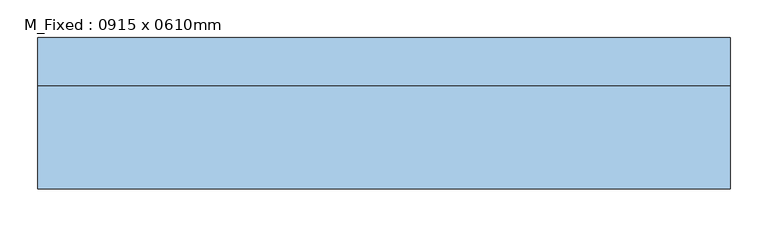
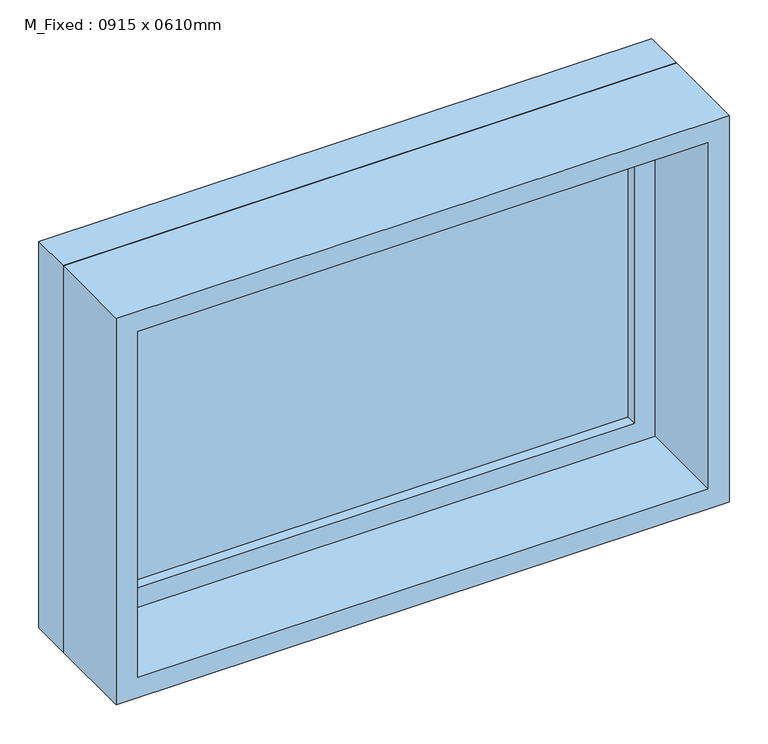
"""IFC4 building model written with IfcOpenShell, lengths in millimetres: window geometry, M_Fixed : 0915 x 0610mm."""

import ifcopenshell
import ifcopenshell.guid

model = None  # the IFC model being written
_history = None  # IfcOwnerHistory: only IFC2X3 demands one
_inside = {}  # id of a spatial element -> (the spatial element, [elements in it])
_under = {}  # id of a project, library or spatial element -> (it, [spatial elements below it])
_declared = {}  # id of a project -> (the project, [libraries it declares])
_typed = {}  # id of a type object -> (the type object, [elements of that type])
_made_of = {}  # id of a material, layer set ... -> (it, [elements and type objects made of it])


def new_model(schema):
    """Start an empty IFC model of exactly this schema.

    Asked for "IFC4X3", IfcOpenShell would pick the latest addendum, in which some entities
    have other attributes; the version numbers below select the first issue.
    IFC2X3 requires an IfcOwnerHistory on every rooted entity: one is made here for all.
    """
    global model, _history
    if schema == "IFC4X3":
        model = ifcopenshell.file(schema_version=(4, 3, 0, 0))
    else:
        model = ifcopenshell.file(schema=schema)
    _inside.clear()
    _under.clear()
    _declared.clear()
    _typed.clear()
    _made_of.clear()
    _history = None
    if model.schema == "IFC2X3":
        org = make("IfcOrganization", Name="unknown")
        user = make(
            "IfcPersonAndOrganization",
            ThePerson=make("IfcPerson", FamilyName="unknown"),
            TheOrganization=org,
        )
        app = make(
            "IfcApplication",
            ApplicationDeveloper=org,
            Version="unknown",
            ApplicationFullName="unknown",
            ApplicationIdentifier="unknown",
        )
        _history = make(
            "IfcOwnerHistory",
            OwningUser=user,
            OwningApplication=app,
            ChangeAction="ADDED",
            CreationDate=0,
        )
    return model


def make(cls, **values):
    """One entity of the class cls with the attributes given. An attribute that is None is left unset."""
    return model.create_entity(
        cls, **{name: value for name, value in values.items() if value is not None}
    )


def rooted(cls, **values):
    """An entity with a GlobalId (a new one), such as an element, a storey or a relation."""
    return make(cls, GlobalId=ifcopenshell.guid.new(), OwnerHistory=_history, **values)


def si_unit(unit_type, name, prefix=None):
    """IfcSIUnit, for example si_unit("LENGTHUNIT", "METRE", prefix="MILLI")."""
    return make("IfcSIUnit", UnitType=unit_type, Prefix=prefix, Name=name)


def assignment(units):
    """IfcUnitAssignment: the units of a project."""
    return None if units is None else make("IfcUnitAssignment", Units=units)


def point(xyz):
    """IfcCartesianPoint."""
    return None if xyz is None else make("IfcCartesianPoint", Coordinates=xyz)


def direction(xyz):
    """IfcDirection."""
    return None if xyz is None else make("IfcDirection", DirectionRatios=xyz)


def frame(location, z_axis=None, x_axis=None):
    """IfcAxis2Placement3D, a coordinate frame: its origin and axes. An axis left out is left unset."""
    return make(
        "IfcAxis2Placement3D",
        Location=point(location),
        Axis=direction(z_axis),
        RefDirection=direction(x_axis),
    )


def origin():
    """The frame at (0, 0, 0) with its axes left unset."""
    return frame((0.0, 0.0, 0.0))


def place(relative_to, where):
    """IfcLocalPlacement: puts the frame where relative to a parent placement (None: the world)."""
    return make(
        "IfcLocalPlacement", PlacementRelTo=relative_to, RelativePlacement=where
    )


def context(
    kind, dimensions, precision=None, world=None, true_north=None, identifier=None
):
    """IfcGeometricRepresentationContext, for example the 3D "Model" context."""
    return make(
        "IfcGeometricRepresentationContext",
        ContextIdentifier=identifier,
        ContextType=kind,
        CoordinateSpaceDimension=dimensions,
        Precision=precision,
        WorldCoordinateSystem=world,
        TrueNorth=true_north,
    )


def project(units=None, contexts=None):
    """IfcProject with its units and contexts."""
    return rooted(
        "IfcProject",
        Name="project",
        RepresentationContexts=contexts,
        UnitsInContext=assignment(units),
    )


def spatial(cls, under=None, at=None, **own):
    """A site, building, storey or space (cls), placed at a placement, below another one or the project."""
    s = rooted(cls, ObjectPlacement=at, **own)
    if under is not None:
        _under.setdefault(under.id(), (under, []))[1].append(s)
    return s


def polyline(points):
    """IfcPolyline through the points."""
    return make("IfcPolyline", Points=[point(p) for p in points])


def outline(outer, holes=None, kind="AREA"):
    """IfcArbitraryClosedProfileDef: a profile drawn as a closed curve; with holes, ...WithVoids."""
    if holes is None:
        return make("IfcArbitraryClosedProfileDef", ProfileType=kind, OuterCurve=outer)
    return make(
        "IfcArbitraryProfileDefWithVoids",
        ProfileType=kind,
        OuterCurve=outer,
        InnerCurves=holes,
    )


def extrude(swept, where, along, depth):
    """IfcExtrudedAreaSolid: the profile swept, set in the frame where, extruded along a direction by depth."""
    return make(
        "IfcExtrudedAreaSolid",
        SweptArea=swept,
        Position=where,
        ExtrudedDirection=direction(along),
        Depth=depth,
    )


def shape(context_of_items, identifier, shape_type, items):
    """IfcShapeRepresentation: the items that make up one representation, for example the "Body"."""
    return make(
        "IfcShapeRepresentation",
        ContextOfItems=context_of_items,
        RepresentationIdentifier=identifier,
        RepresentationType=shape_type,
        Items=items,
    )


def source(mapping_origin, context_of_items, identifier, shape_type, items):
    """IfcRepresentationMap: a shape defined once, which mapped items show again and again."""
    return make(
        "IfcRepresentationMap",
        MappingOrigin=mapping_origin,
        MappedRepresentation=shape(context_of_items, identifier, shape_type, items),
    )


def transform(
    local_origin,
    x_axis=None,
    y_axis=None,
    z_axis=None,
    scale=None,
    scale2=None,
    scale3=None,
    uniform=True,
):
    """IfcCartesianTransformationOperator3D, or its non-uniform kind. x_axis, y_axis, z_axis: its Axis1, 2, 3."""
    if uniform:
        return make(
            "IfcCartesianTransformationOperator3D",
            Axis1=direction(x_axis),
            Axis2=direction(y_axis),
            LocalOrigin=point(local_origin),
            Scale=scale,
            Axis3=direction(z_axis),
        )
    return make(
        "IfcCartesianTransformationOperator3DnonUniform",
        Axis1=direction(x_axis),
        Axis2=direction(y_axis),
        LocalOrigin=point(local_origin),
        Scale=scale,
        Axis3=direction(z_axis),
        Scale2=scale2,
        Scale3=scale3,
    )


def mapped(mapping_source, mapping_target):
    """IfcMappedItem: shows the shape of a source again, moved by a transform."""
    return make(
        "IfcMappedItem", MappingSource=mapping_source, MappingTarget=mapping_target
    )


def made_of(thing, what):
    """Note that an element or type object is made of a material, layer set ...; save() writes the relation."""
    if what is not None:
        _made_of.setdefault(what.id(), (what, []))[1].append(thing)
    return thing


def element(
    cls,
    number,
    at=None,
    inside=None,
    cuts=None,
    type_object=None,
    material=None,
    context=None,
    identifier="Body",
    shape_type=None,
    held_by="IfcProductDefinitionShape",
    body=None,
    shapes=None,
    **own,
):
    """One element of the class cls, such as IfcWall. Its Tag is "e" and its number.

    at: its placement. inside: the storey or other place that contains it. cuts: it is an
    opening in that element (IfcRelVoidsElement). A single representation is given by context,
    identifier, shape_type and body (its items); several are given by shapes. held_by: the class
    of the entity that holds the representations. save() writes the other relations.
    """
    e = rooted(cls, Tag="e%d" % number, ObjectPlacement=at, **own)
    if body is not None:
        shapes = [shape(context, identifier, shape_type, body)]
    if shapes is not None:
        e.Representation = make(held_by, Representations=shapes)
    if inside is not None:
        _inside.setdefault(inside.id(), (inside, []))[1].append(e)
    if cuts is not None:
        rooted(
            "IfcRelVoidsElement", RelatingBuildingElement=cuts, RelatedOpeningElement=e
        )
    if type_object is not None:
        _typed.setdefault(type_object.id(), (type_object, []))[1].append(e)
    return made_of(e, material)


def aggregate(whole, parts):
    """IfcRelAggregates: a whole, such as a stair, and the parts it consists of."""
    return rooted("IfcRelAggregates", RelatingObject=whole, RelatedObjects=parts)


def save(model, path):
    """Write the relations noted so far, then the file.

    IfcRelAggregates (storeys below a building ...), IfcRelContainedInSpatialStructure (elements
    in a storey), IfcRelDefinesByType, IfcRelAssociatesMaterial and IfcRelDeclares: one each for
    every whole, place, type object, material and project.
    """
    for whole, parts in _under.values():
        aggregate(whole, parts)
    for where, things in _inside.values():
        rooted(
            "IfcRelContainedInSpatialStructure",
            RelatedElements=things,
            RelatingStructure=where,
        )
    for kind, things in _typed.values():
        rooted("IfcRelDefinesByType", RelatedObjects=things, RelatingType=kind)
    for what, things in _made_of.values():
        rooted("IfcRelAssociatesMaterial", RelatedObjects=things, RelatingMaterial=what)
    for by, libraries in _declared.values():
        rooted("IfcRelDeclares", RelatingContext=by, RelatedDefinitions=libraries)
    model.write(path)


def m_fixed_0915_x_0610mm_70a843a6(model_context):
    return source(origin(), model_context, "Body", "SweptSolid", [
        extrude(outline(polyline([(-394.5, 78.0), (394.5, 78.0), (394.5, 66.0), (-394.5, 66.0), (-394.5, 78.0)])), frame((0.0, 0.0, 978.0), z_axis=(0.0, 0.0, 1.0), x_axis=(1.0, 0.0, 0.0)), (0.0, 0.0, 1.0), 484.0),
        extrude(outline(polyline([(1506.0, -438.5), (934.0, -438.5), (934.0, 438.5), (1506.0, 438.5), (1506.0, -438.5)]), holes=[polyline([(1462.0, -394.5), (1462.0, 394.5), (978.0, 394.5), (978.0, -394.5), (1462.0, -394.5)])]), frame((0.0, 50.0, 0.0), z_axis=(0.0, 1.0, 0.0), x_axis=(0.0, 0.0, 1.0)), (0.0, 0.0, 1.0), 44.0),
        extrude(outline(polyline([(1525.0, -457.5), (915.0, -457.5), (915.0, 457.5), (1525.0, 457.5), (1525.0, -457.5)]), holes=[polyline([(1506.0, -438.5), (1506.0, 438.5), (934.0, 438.5), (934.0, -438.5), (1506.0, -438.5)])]), frame((0.0, 50.0, 0.0), z_axis=(0.0, 1.0, 0.0), x_axis=(0.0, 0.0, 1.0)), (0.0, 0.0, 1.0), 63.0),
        extrude(outline(polyline([(1525.0, -457.5), (915.0, -457.5), (915.0, 457.5), (1525.0, 457.5), (1525.0, -457.5)]), holes=[polyline([(1493.0, -425.5), (1493.0, 425.5), (947.0, 425.5), (947.0, -425.5), (1493.0, -425.5)])]), frame((0.0, -87.0, 0.0), z_axis=(0.0, 1.0, 0.0), x_axis=(0.0, 0.0, 1.0)), (0.0, 0.0, 1.0), 137.0),
    ])


if __name__ == "__main__":
    model = new_model("IFC4")
    model_context = context("Model", 3, world=origin())
    ifc_project = project(units=[si_unit("LENGTHUNIT", "METRE", prefix="MILLI")], contexts=[model_context])
    site = spatial("IfcSite", under=ifc_project)
    building = spatial("IfcBuilding", under=site)
    placement = place(None, origin())
    m_fixed_0915_x_0610mm_shape = m_fixed_0915_x_0610mm_70a843a6(model_context)
    element("IfcWindow", 1, ObjectType="M_Fixed : 0915 x 0610mm", at=placement, inside=building, context=model_context, shape_type="MappedRepresentation", body=[
        mapped(m_fixed_0915_x_0610mm_shape, transform((0.0, 0.0, 0.0), x_axis=(1.0, 0.0, 0.0), y_axis=(0.0, 1.0, 0.0), z_axis=(0.0, 0.0, 1.0))),
    ])
    save(model, "model.ifc")

# Revit data of these elements
# Project information
#   Project Issue Date = "Issue Date"
#   Project Status = "Project Status"
#   Client Name = "Owner"
#   Project Address = "Enter address here"
#   Project Name = "Project Name"
#   Project Number = "0001"
# Type "M_Fixed : 0915 x 0610mm"
#   Type Mark = "14"
#   Construction Type Id = "GSP4R"
#   Analytic Construction = "1/8 in Pilkington single glazing"
#   Visual Light Transmittance = 0.9
#   Thermal Resistance (R) = 0.271106 (m²·K)/W
#   Solar Heat Gain Coefficient = 0.78
#   Heat Transfer Coefficient (U) = 3.6886 W/(m²·K)
#   Height = 610 mm
#   Default Sill Height = 915 mm
#   Width = 915 mm
#   Window Inset = 19 mm
#   Frame Exterior Material = Sash
#   Frame Interior Material = Sash
#   Glass Pane Material = Glass
#   Sash = Sash
#   Wall Closure = (empty or 0)
# Element 1 (IfcWindow, "M_Fixed : 0915 x 0610mm")
#   Materials on its faces: "Sash", "Glass"
# Materials
#   "Sash": class "Wood", colour RGB 224 178 126, transparency 0, Cost = 0
#   "Glass": class "Glass", colour RGB 0 128 192, transparency 0.9, Description = "Soda Lime Glass", Cost = 0
